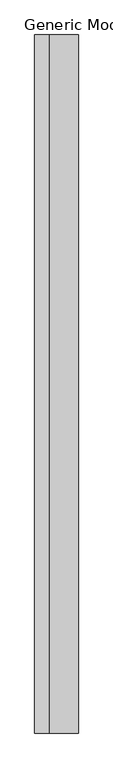
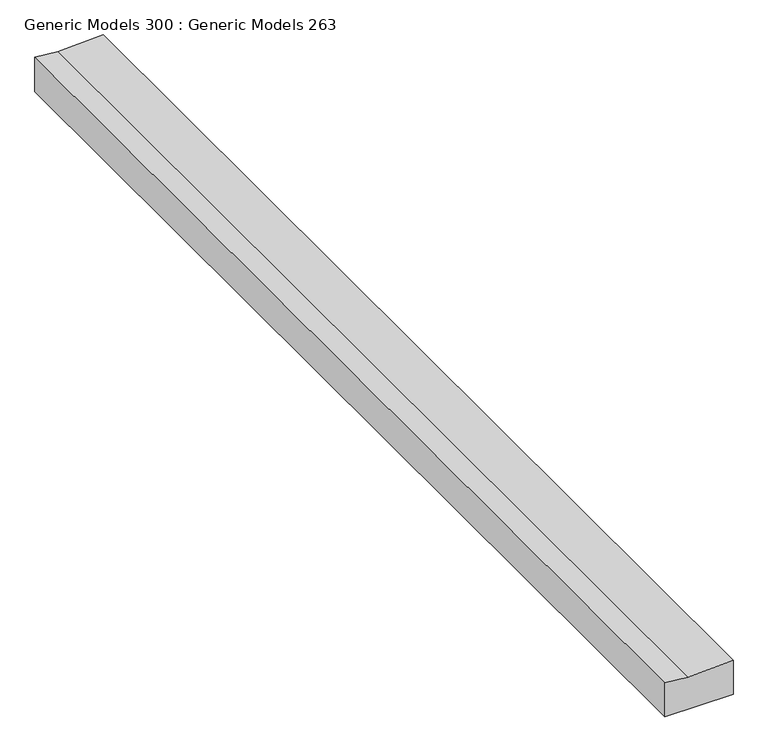
"""IFC4 building model written with IfcOpenShell, lengths in millimetres: proxy geometry, Generic Models 300 : Generic Models 263."""

from ifc_helpers import new_model, si_unit, frame, origin, place, context, project, spatial, polyline, outline, extrude, source, transform, mapped, element, save


def generic_models_300_generic_models_263_12a764e5(model_context):
    return source(origin(), model_context, "Body", "SweptSolid", [
        extrude(outline(polyline([(-139.1379392, 91579.9797726), (-381.0, 91579.9797726), (-381.0, 92037.1797726), (-139.7, 92037.1797726), (-152.4, 91732.3797726), (-139.1379392, 91579.9797726)])), frame((0.0, -6732.6272578, 0.0), z_axis=(0.0, 1.0, 0.0), x_axis=(0.0, 0.0, 1.0)), (0.0, 0.0, 1.0), 7315.2),
    ])


if __name__ == "__main__":
    model = new_model("IFC4")
    model_context = context("Model", 3, world=origin())
    ifc_project = project(units=[si_unit("LENGTHUNIT", "METRE", prefix="MILLI")], contexts=[model_context])
    site = spatial("IfcSite", under=ifc_project)
    building = spatial("IfcBuilding", under=site)
    placement = place(None, origin())
    generic_models_300_generic_models_263_shape = generic_models_300_generic_models_263_12a764e5(model_context)
    element("IfcBuildingElementProxy", 1, Name="Generic Models 300 : Generic Models 263", ObjectType="Generic Models 300 : Generic Models 263", at=placement, inside=building, context=model_context, shape_type="MappedRepresentation", body=[
        mapped(generic_models_300_generic_models_263_shape, transform((0.0, 0.0, 0.0), x_axis=(1.0, 0.0, 0.0), y_axis=(0.0, 1.0, 0.0), z_axis=(0.0, 0.0, 1.0))),
    ])
    save(model, "model.ifc")

# Revit data of these elements
# Element 1 (IfcBuildingElementProxy, "Generic Models 300 : Generic Models 263")
#   Materials on its faces: "CONCRETE CURB"
# Materials
#   "CONCRETE CURB": class "Concrete", colour RGB 191 191 191, transparency 0, Description = "Cast-in-place concrete", Cost = 0
